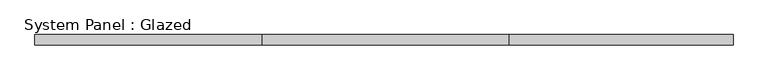
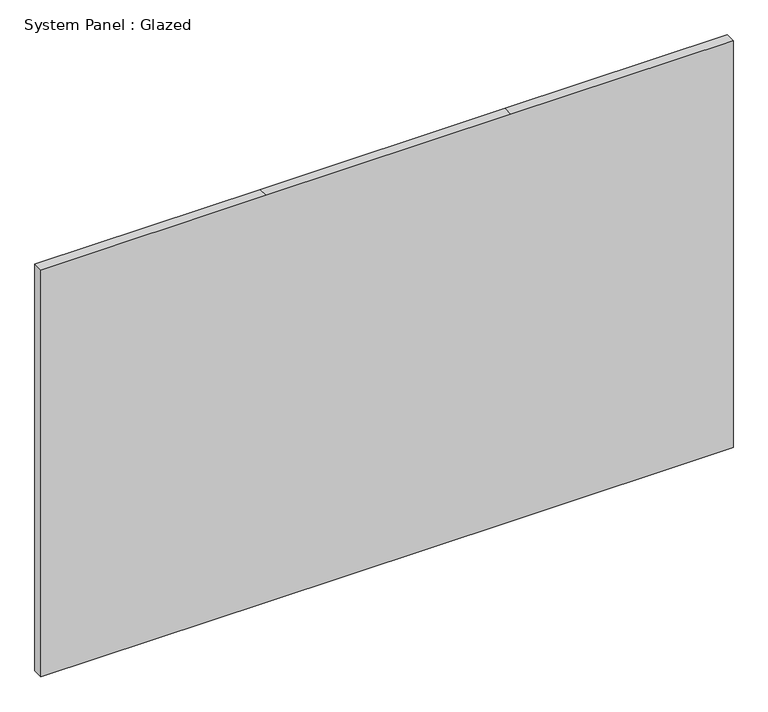
"""IFC4 building model written with IfcOpenShell, lengths in millimetres: plate geometry, System Panel : Glazed."""

from ifc_helpers import new_model, si_unit, frame, origin, place, context, project, spatial, polyline, outline, extrude, source, transform, mapped, element, save


def system_panel_glazed_db19d737(model_context):
    return source(origin(), model_context, "Body", "SweptSolid", [
        extrude(outline(polyline([(0.0, -1696.5), (0.0, -592.5), (0.0, 607.5), (0.0, 1696.5), (2110.0, 1696.5), (2110.0, 607.5), (2110.0, -592.5), (2110.0, -1696.5), (0.0, -1696.5)])), frame((0.0, -25.0, 0.0), z_axis=(0.0, 1.0, 0.0), x_axis=(0.0, 0.0, 1.0)), (0.0, 0.0, 1.0), 50.0),
    ])


if __name__ == "__main__":
    model = new_model("IFC4")
    model_context = context("Model", 3, world=origin())
    ifc_project = project(units=[si_unit("LENGTHUNIT", "METRE", prefix="MILLI")], contexts=[model_context])
    site = spatial("IfcSite", under=ifc_project)
    building = spatial("IfcBuilding", under=site)
    placement = place(None, origin())
    system_panel_glazed_shape = system_panel_glazed_db19d737(model_context)
    element("IfcPlate", 1, ObjectType="System Panel : Glazed", at=placement, inside=building, context=model_context, shape_type="MappedRepresentation", body=[
        mapped(system_panel_glazed_shape, transform((0.0, 0.0, 0.0), x_axis=(1.0, 0.0, 0.0), y_axis=(0.0, 1.0, 0.0), z_axis=(0.0, 0.0, 1.0))),
    ])
    save(model, "model.ifc")

# Revit data of these elements
# Type "System Panel : Glazed"
#   Type Mark = "CW-GLASS"
# Element 1 (IfcPlate, "System Panel : Glazed")
#   Materials on its faces: "Glass_Clear"
# Materials
#   "Glass_Clear": class "Glass", colour RGB 128 128 255, transparency 0.8, Comments = "Rendering appearance not upgraded ", Cost = 0
